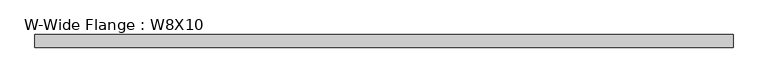
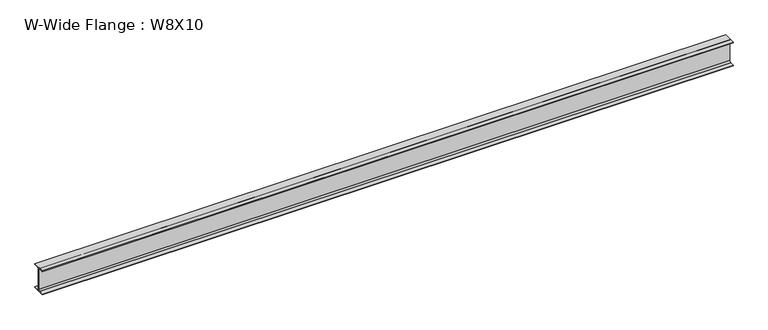
"""IFC4 building model written with IfcOpenShell, lengths in millimetres: beam geometry, W-Wide Flange : W8X10."""

from ifc_helpers import new_model, si_unit, point, frame, frame_2d, origin, place, context, project, spatial, polyline, circle_curve, trimmed, segment, composite_curve, outline, extrude, source, transform, mapped, element, save


def w_wide_flange_w8x10_418ab950(model_context):
    return source(origin(), model_context, "Body", "SweptSolid", [
        extrude(outline(composite_curve([segment(polyline([(50.038, -94.996), (50.038, -100.203), (-50.038, -100.203), (-50.038, -94.996), (-14.4145, -94.996)]), True, "CONTINUOUS"), segment(trimmed(circle_curve(frame_2d((-14.4145, -82.7405)), 12.2555), [point((-14.4145, -94.996))], [point((-2.159, -82.7405))], True, "CARTESIAN"), True, "CONTINUOUS"), segment(polyline([(-2.159, -82.7405), (-2.159, 82.7405)]), True, "CONTINUOUS"), segment(trimmed(circle_curve(frame_2d((-14.4145, 82.7405)), 12.2555), [point((-2.159, 82.7405))], [point((-14.4145, 94.996))], True, "CARTESIAN"), True, "CONTINUOUS"), segment(polyline([(-14.4145, 94.996), (-50.038, 94.996), (-50.038, 100.203), (50.038, 100.203), (50.038, 94.996), (14.4145, 94.996)]), True, "CONTINUOUS"), segment(trimmed(circle_curve(frame_2d((14.4145, 82.7405)), 12.2555), [point((14.4145, 94.996))], [point((2.159, 82.7405))], True, "CARTESIAN"), True, "CONTINUOUS"), segment(polyline([(2.159, 82.7405), (2.159, -82.7405)]), True, "CONTINUOUS"), segment(trimmed(circle_curve(frame_2d((14.4145, -82.7405)), 12.2555), [point((2.159, -82.7405))], [point((14.4145, -94.996))], True, "CARTESIAN"), True, "CONTINUOUS"), segment(polyline([(14.4145, -94.996), (50.038, -94.996)]), True, "CONTINUOUS")], self_intersect=False)), frame((-2769.4255, 0.0, 0.0), z_axis=(1.0, 0.0, 0.0), x_axis=(0.0, 1.0, 0.0)), (0.0, 0.0, 1.0), 5514.1633906),
    ])


if __name__ == "__main__":
    model = new_model("IFC4")
    model_context = context("Model", 3, world=origin())
    ifc_project = project(units=[si_unit("LENGTHUNIT", "METRE", prefix="MILLI")], contexts=[model_context])
    site = spatial("IfcSite", under=ifc_project)
    building = spatial("IfcBuilding", under=site)
    placement = place(None, origin())
    w_wide_flange_w8x10_shape = w_wide_flange_w8x10_418ab950(model_context)
    element("IfcBeam", 1, ObjectType="W-Wide Flange : W8X10", at=placement, inside=building, context=model_context, shape_type="MappedRepresentation", body=[
        mapped(w_wide_flange_w8x10_shape, transform((0.0, 0.0, 0.0), x_axis=(1.0, 0.0, 0.0), y_axis=(0.0, 1.0, 0.0), z_axis=(0.0, 0.0, 1.0))),
    ])
    save(model, "model.ifc")

# Revit data of these elements
# Type "W-Wide Flange : W8X10"
#   Assembly Code = "B10"
#   W = 10
#   Length [instance default] = 1524 mm
#   bf = 100.076 mm
#   d = 200.406 mm
#   k = 17.463 mm
#   k2 = 12.255 mm
#   tf = 5.207 mm
#   tw = 4.318 mm
#   A = 0.00190967 m²
#   Structural Material [instance default] = Steel ASTM A992
# Element 1 (IfcBeam, "W-Wide Flange : W8X10")
#   Structural Material = Aluminum, Anodized Red
#   Materials on its faces: "Aluminum, Anodized Red"
# Materials
#   "Steel ASTM A992": class "Metal", colour RGB 128 0 0, transparency 0, Description = "Structural steel 50ksi", Cost = 0
#   "Aluminum, Anodized Red": class "Metal", colour RGB 120 120 120, transparency 0, Description = "Anodized aluminum, red", Cost = 0
